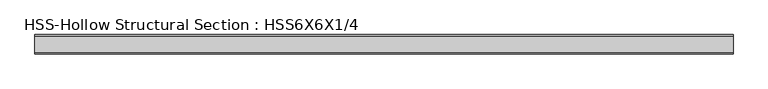
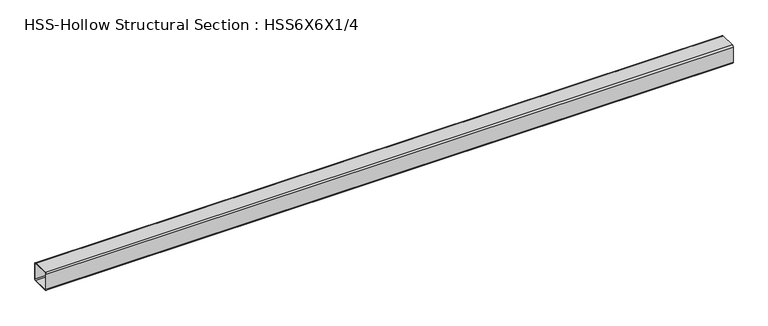
"""IFC4 building model written with IfcOpenShell, lengths in millimetres: beam geometry, HSS-Hollow Structural Section : HSS6X6X1/4."""

from ifc_helpers import new_model, si_unit, point, frame, frame_2d, origin, place, context, project, spatial, polyline, circle_curve, trimmed, segment, composite_curve, outline, extrude, source, transform, mapped, element, save


def hss_hollow_structural_section_hss6x6x1_4_f83ef3ea(model_context):
    return source(origin(), model_context, "Body", "SweptSolid", [
        extrude(outline(composite_curve([segment(polyline([(76.2, 64.3636), (76.2, -64.3636)]), True, "CONTINUOUS"), segment(trimmed(circle_curve(frame_2d((64.3636, -64.3636)), 11.8364), [point((76.2, -64.3636))], [point((64.3636, -76.2))], False, "CARTESIAN"), True, "CONTINUOUS"), segment(polyline([(64.3636, -76.2), (-64.3636, -76.2)]), True, "CONTINUOUS"), segment(trimmed(circle_curve(frame_2d((-64.3636, -64.3636)), 11.8364), [point((-64.3636, -76.2))], [point((-76.2, -64.3636))], False, "CARTESIAN"), True, "CONTINUOUS"), segment(polyline([(-76.2, -64.3636), (-76.2, 64.3636)]), True, "CONTINUOUS"), segment(trimmed(circle_curve(frame_2d((-64.3636, 64.3636)), 11.8364), [point((-76.2, 64.3636))], [point((-64.3636, 76.2))], False, "CARTESIAN"), True, "CONTINUOUS"), segment(polyline([(-64.3636, 76.2), (64.3636, 76.2)]), True, "CONTINUOUS"), segment(trimmed(circle_curve(frame_2d((64.3636, 64.3636)), 11.8364), [point((64.3636, 76.2))], [point((76.2, 64.3636))], False, "CARTESIAN"), True, "CONTINUOUS")], self_intersect=False), holes=[composite_curve([segment(trimmed(circle_curve(frame_2d((-64.3636, 64.3636)), 5.9182), [point((-64.3636, 70.2818))], [point((-70.2818, 64.3636))], True, "CARTESIAN"), True, "CONTINUOUS"), segment(polyline([(-70.2818, 64.3636), (-70.2818, -64.3636)]), True, "CONTINUOUS"), segment(trimmed(circle_curve(frame_2d((-64.3636, -64.3636)), 5.9182), [point((-70.2818, -64.3636))], [point((-64.3636, -70.2818))], True, "CARTESIAN"), True, "CONTINUOUS"), segment(polyline([(-64.3636, -70.2818), (64.3636, -70.2818)]), True, "CONTINUOUS"), segment(trimmed(circle_curve(frame_2d((64.3636, -64.3636)), 5.9182), [point((64.3636, -70.2818))], [point((70.2818, -64.3636))], True, "CARTESIAN"), True, "CONTINUOUS"), segment(polyline([(70.2818, -64.3636), (70.2818, 64.3636)]), True, "CONTINUOUS"), segment(trimmed(circle_curve(frame_2d((64.3636, 64.3636)), 5.9182), [point((70.2818, 64.3636))], [point((64.3636, 70.2818))], True, "CARTESIAN"), True, "CONTINUOUS"), segment(polyline([(64.3636, 70.2818), (-64.3636, 70.2818)]), True, "CONTINUOUS")], self_intersect=False)]), frame((-2751.100302, 0.0, 0.0), z_axis=(1.0, 0.0, 0.0), x_axis=(0.0, 1.0, 0.0)), (0.0, 0.0, 1.0), 5507.000302),
    ])


if __name__ == "__main__":
    model = new_model("IFC4")
    model_context = context("Model", 3, world=origin())
    ifc_project = project(units=[si_unit("LENGTHUNIT", "METRE", prefix="MILLI")], contexts=[model_context])
    site = spatial("IfcSite", under=ifc_project)
    building = spatial("IfcBuilding", under=site)
    placement = place(None, origin())
    hss_hollow_structural_section_hss6x6x1_4_shape = hss_hollow_structural_section_hss6x6x1_4_f83ef3ea(model_context)
    element("IfcBeam", 1, ObjectType="HSS-Hollow Structural Section : HSS6X6X1/4", at=placement, inside=building, context=model_context, shape_type="MappedRepresentation", body=[
        mapped(hss_hollow_structural_section_hss6x6x1_4_shape, transform((0.0, 0.0, 0.0), x_axis=(1.0, 0.0, 0.0), y_axis=(0.0, 1.0, 0.0), z_axis=(0.0, 0.0, 1.0))),
    ])
    save(model, "model.ifc")

# Revit data of these elements
# Type "HSS-Hollow Structural Section : HSS6X6X1/4"
#   Assembly Code = "B10"
#   Shape = "Square"
#   W = 19
#   Ht = 0' - 6"
#   Length [instance default] = 5' - 0"
#   b = 0' - 6"
#   kr = 0' - 0.466"
#   t = 0' - 0.233"
#   A = 0.0363889 SF
#   Structural Material [instance default] = Steel ASTM A500, Grade B, Rectangular and Square
# Element 1 (IfcBeam, "HSS-Hollow Structural Section : HSS6X6X1/4")
#   Materials on its faces: "Steel ASTM A500, Grade B, Rectangular and Square"
# Materials
#   "Steel ASTM A500, Grade B, Rectangular and Square": class "Metal", colour RGB 199 199 199, transparency 0, Description = "Carbon steel", Cost = 0
